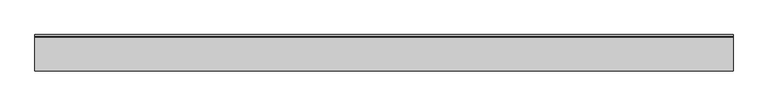
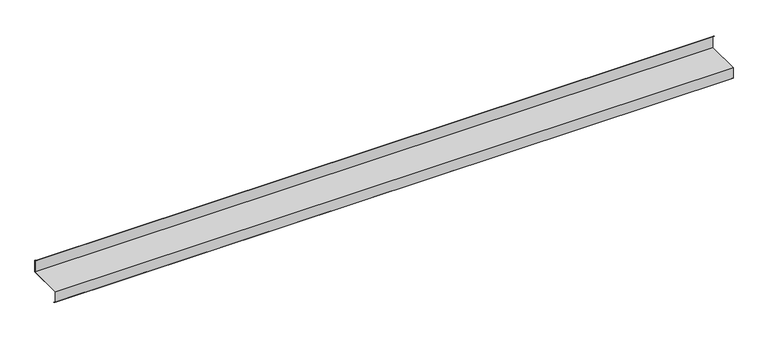
"""IFC4 building model written with IfcOpenShell, lengths in millimetres: proxy geometry, Generic Models 7:Generic Models 1:337419:Generic Models 1:337419 : Generic Models 7:Generic Models 1:337419:11 : Generic Models 7:Generic Models 1:337419:Generic Models 1:337419 : Generic Models 7:Generic Models 1:337419:301336."""

from ifc_helpers import new_model, si_unit, frame, origin, place, context, project, spatial, polyline, outline, extrude, source, transform, mapped, element, save


def generic_models_a01c26df(model_context):
    return source(origin(), model_context, "Body", "SweptSolid", [
        extrude(outline(polyline([(-567932.6413841, 6126.1625), (-568183.8632591, 6126.1625), (-568183.8632591, 6050.861086), (-568170.0763026, 6039.2924559), (-568172.0482374, 6037.320521), (-568186.6413841, 6049.565625), (-568186.6413841, 6128.940625), (-567935.4195091, 6128.940625), (-567935.4195091, 6210.592039), (-567949.0202751, 6222.0044367), (-567947.0483402, 6223.9763716), (-567932.6413841, 6211.8875), (-567932.6413841, 6126.1625)])), frame((591306.0367242, 0.0, 0.0), z_axis=(1.0, 0.0, 0.0), x_axis=(0.0, 1.0, 0.0)), (0.0, 0.0, 1.0), 4876.8),
    ])


if __name__ == "__main__":
    model = new_model("IFC4")
    model_context = context("Model", 3, world=origin())
    ifc_project = project(units=[si_unit("LENGTHUNIT", "METRE", prefix="MILLI")], contexts=[model_context])
    site = spatial("IfcSite", under=ifc_project)
    building = spatial("IfcBuilding", under=site)
    placement = place(None, origin())
    generic_models_shape = generic_models_a01c26df(model_context)
    element("IfcBuildingElementProxy", 1, Name="Generic Models 7:Generic Models 1:337419:Generic Models 1:337419 : Generic Models 7:Generic Models 1:337419:11 : Generic Models 7:Generic Models 1:337419:Generic Models 1:337419 : Generic Models 7:Generic Models 1:337419:301336", ObjectType="Generic Models 7:Generic Models 1:337419:Generic Models 1:337419 : Generic Models 7:Generic Models 1:337419:11 : Generic Models 7:Generic Models 1:337419:Generic Models 1:337419 : Generic Models 7:Generic Models 1:337419:301336", at=placement, inside=building, context=model_context, shape_type="MappedRepresentation", body=[
        mapped(generic_models_shape, transform((0.0, 0.0, 0.0), x_axis=(1.0, 0.0, 0.0), y_axis=(0.0, 1.0, 0.0), z_axis=(0.0, 0.0, 1.0))),
    ])
    save(model, "model.ifc")

# Revit data of these elements
# Type "Generic Models 7:Generic Models 1:337419:Generic Models 1:337419 : Generic Models 7:Generic Models 1:337419:11 : Generic Models 7:Generic Models 1:337419:Generic Models 1:337419 : Generic Models 7:Generic Models 1:337419:301336"
#   NameOverride = "Generic Models 7:Generic Models 1:337419:Generic Models 1:337419 : Generic Models 7:Generic Models 1:337419:301336"
#   ObjectTypeOverride = "Generic Models 1:337419 : Generic Models 7:Generic Models 1:337419"
#   Reference = "Generic Models 1"
#   Tag = "301336"
# Element 1 (IfcBuildingElementProxy, "Generic Models 7:Generic Models 1:337419:Generic Models 1:337419 : Generic Models 7:Generic Models 1:337419:11 : Generic Models 7:Generic Models 1:337419:Generic Models 1:337419 : Generic Models 7:Generic Models 1:337419:301336")
#   Materials on its faces: "'ZEE' SECTION (8.0x3.5Z - SEE STRUCT. DWGS)"
# Materials
#   "'ZEE' SECTION (8.0x3.5Z - SEE STRUCT. DWGS)": class "Unassigned", colour RGB 210 209 208, transparency 0, Keynote = "M05121300.02", Cost = 0
